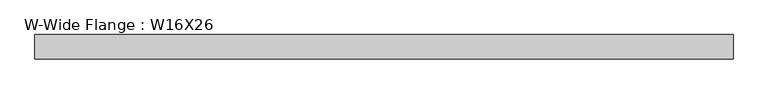
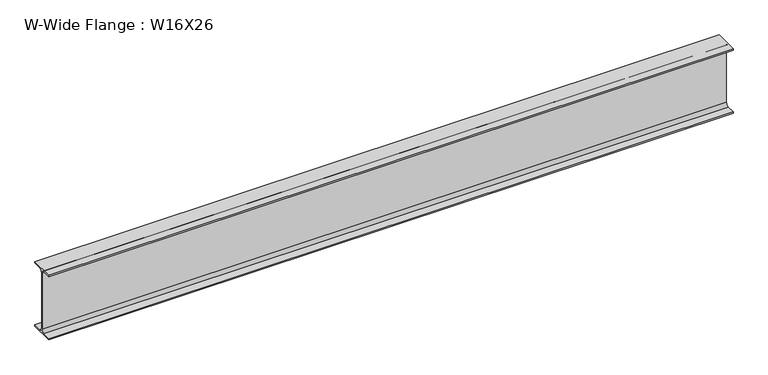
"""IFC4 building model written with IfcOpenShell, lengths in millimetres: beam geometry, W-Wide Flange : W16X26."""

from ifc_helpers import new_model, si_unit, point, frame, frame_2d, origin, place, context, project, spatial, polyline, circle_curve, trimmed, segment, composite_curve, outline, extrude, source, transform, mapped, element, save


def w_wide_flange_w16x26_e7c4c9f7(model_context):
    return source(origin(), model_context, "Body", "SweptSolid", [
        extrude(outline(composite_curve([segment(polyline([(-69.85, -190.5496094), (-21.43125, -190.5496094)]), True, "CONTINUOUS"), segment(trimmed(circle_curve(frame_2d((-21.43125, -172.2933594)), 18.25625), [point((-21.43125, -190.5496094))], [point((-3.175, -172.2933594))], True, "CARTESIAN"), True, "CONTINUOUS"), segment(polyline([(-3.175, -172.2933594), (-3.175, 172.2933594)]), True, "CONTINUOUS"), segment(trimmed(circle_curve(frame_2d((-21.43125, 172.2933594)), 18.25625), [point((-3.175, 172.2933594))], [point((-21.43125, 190.5496094))], True, "CARTESIAN"), True, "CONTINUOUS"), segment(polyline([(-21.43125, 190.5496094), (-69.85, 190.5496094), (-69.85, 199.2808594), (69.85, 199.2808594), (69.85, 190.5496094), (21.43125, 190.5496094)]), True, "CONTINUOUS"), segment(trimmed(circle_curve(frame_2d((21.43125, 172.2933594)), 18.25625), [point((21.43125, 190.5496094))], [point((3.175, 172.2933594))], True, "CARTESIAN"), True, "CONTINUOUS"), segment(polyline([(3.175, 172.2933594), (3.175, -172.2933594)]), True, "CONTINUOUS"), segment(trimmed(circle_curve(frame_2d((21.43125, -172.2933594)), 18.25625), [point((3.175, -172.2933594))], [point((21.43125, -190.5496094))], True, "CARTESIAN"), True, "CONTINUOUS"), segment(polyline([(21.43125, -190.5496094), (69.85, -190.5496094), (69.85, -199.2808594), (-69.85, -199.2808594), (-69.85, -190.5496094)]), True, "CONTINUOUS")], self_intersect=False)), frame((-1993.9, 0.0, 0.0), z_axis=(1.0, 0.0, 0.0), x_axis=(0.0, 1.0, 0.0)), (0.0, 0.0, 1.0), 3987.8),
    ])


if __name__ == "__main__":
    model = new_model("IFC4")
    model_context = context("Model", 3, world=origin())
    ifc_project = project(units=[si_unit("LENGTHUNIT", "METRE", prefix="MILLI")], contexts=[model_context])
    site = spatial("IfcSite", under=ifc_project)
    building = spatial("IfcBuilding", under=site)
    placement = place(None, origin())
    w_wide_flange_w16x26_shape = w_wide_flange_w16x26_e7c4c9f7(model_context)
    element("IfcBeam", 1, ObjectType="W-Wide Flange : W16X26", at=placement, inside=building, context=model_context, shape_type="MappedRepresentation", body=[
        mapped(w_wide_flange_w16x26_shape, transform((0.0, 0.0, 0.0), x_axis=(1.0, 0.0, 0.0), y_axis=(0.0, 1.0, 0.0), z_axis=(0.0, 0.0, 1.0))),
    ])
    save(model, "model.ifc")

# Revit data of these elements
# Type "W-Wide Flange : W16X26"
#   Assembly Code = "B10"
#   W = 26
#   Start Extension Calculation [instance default] = 10' - 0"
#   Start Extension [instance default] = -0' - 0 1/2"
#   End Extension Calculation [instance default] = 10' - 0"
#   End Extension [instance default] = -0' - 0 1/2"
#   Length [instance default] = 5' - 0"
#   bf = 0' - 5 1/2"
#   d = 1' - 3 177/256"
#   k = 0' - 1 1/16"
#   k2 = 0' - 0 23/32"
#   tf = 0' - 0 11/32"
#   tw = 0' - 0 1/4"
#   A = 0.05 SF
#   Beam Material [instance default] = Metal - Steel - ASTM A992
# Element 1 (IfcBeam, "W-Wide Flange : W16X26")
#   Materials on its faces: "Metal - Steel - ASTM A992"
# Materials
#   "Metal - Steel - ASTM A992": class "Metal", colour RGB 128 0 0, transparency 0
